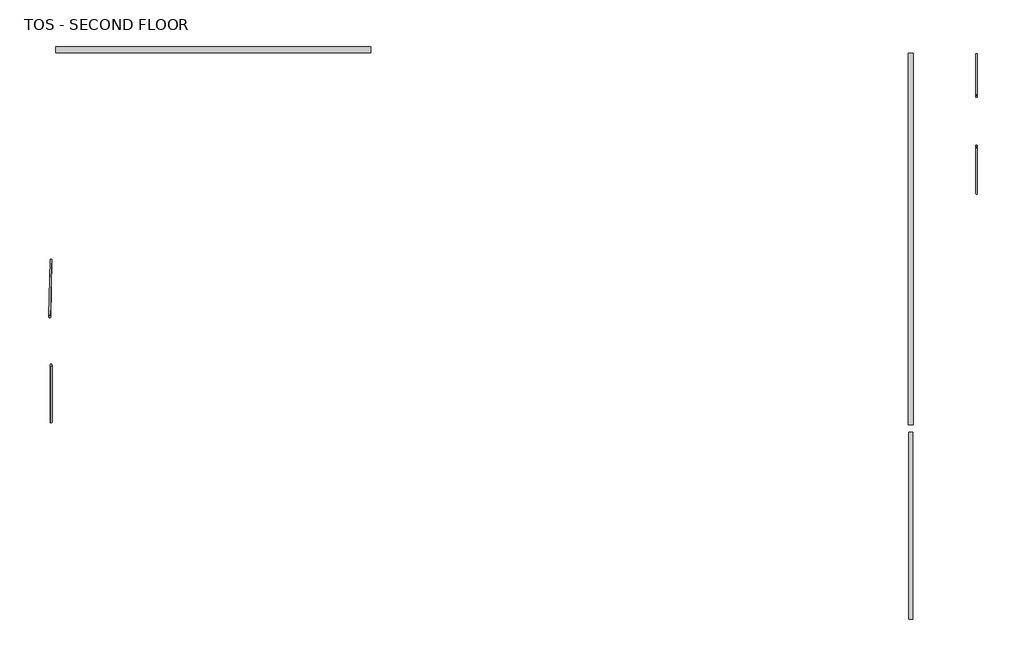
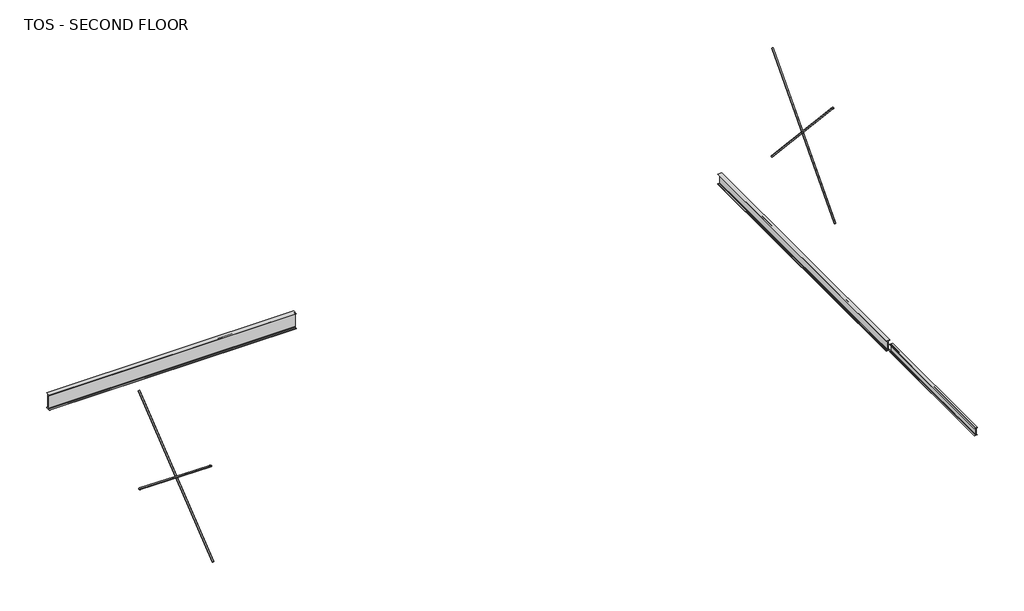
# One storey: 4 members, 3 beams.
"""IFC4 building model written with IfcOpenShell, lengths in millimetres."""

import ifcopenshell
import ifcopenshell.guid

model = None  # the IFC model being written
_history = None  # IfcOwnerHistory: only IFC2X3 demands one
_inside = {}  # id of a spatial element -> (the spatial element, [elements in it])
_under = {}  # id of a project, library or spatial element -> (it, [spatial elements below it])
_declared = {}  # id of a project -> (the project, [libraries it declares])
_typed = {}  # id of a type object -> (the type object, [elements of that type])
_made_of = {}  # id of a material, layer set ... -> (it, [elements and type objects made of it])


def new_model(schema):
    """Start an empty IFC model of exactly this schema.

    Asked for "IFC4X3", IfcOpenShell would pick the latest addendum, in which some entities
    have other attributes; the version numbers below select the first issue.
    IFC2X3 requires an IfcOwnerHistory on every rooted entity: one is made here for all.
    """
    global model, _history
    if schema == "IFC4X3":
        model = ifcopenshell.file(schema_version=(4, 3, 0, 0))
    else:
        model = ifcopenshell.file(schema=schema)
    _inside.clear()
    _under.clear()
    _declared.clear()
    _typed.clear()
    _made_of.clear()
    _history = None
    if model.schema == "IFC2X3":
        org = make("IfcOrganization", Name="unknown")
        user = make(
            "IfcPersonAndOrganization",
            ThePerson=make("IfcPerson", FamilyName="unknown"),
            TheOrganization=org,
        )
        app = make(
            "IfcApplication",
            ApplicationDeveloper=org,
            Version="unknown",
            ApplicationFullName="unknown",
            ApplicationIdentifier="unknown",
        )
        _history = make(
            "IfcOwnerHistory",
            OwningUser=user,
            OwningApplication=app,
            ChangeAction="ADDED",
            CreationDate=0,
        )
    return model


def make(cls, **values):
    """One entity of the class cls with the attributes given. An attribute that is None is left unset."""
    return model.create_entity(
        cls, **{name: value for name, value in values.items() if value is not None}
    )


def rooted(cls, **values):
    """An entity with a GlobalId (a new one), such as an element, a storey or a relation."""
    return make(cls, GlobalId=ifcopenshell.guid.new(), OwnerHistory=_history, **values)


def si_unit(unit_type, name, prefix=None):
    """IfcSIUnit, for example si_unit("LENGTHUNIT", "METRE", prefix="MILLI")."""
    return make("IfcSIUnit", UnitType=unit_type, Prefix=prefix, Name=name)


def assignment(units):
    """IfcUnitAssignment: the units of a project."""
    return None if units is None else make("IfcUnitAssignment", Units=units)


def point(xyz):
    """IfcCartesianPoint."""
    return None if xyz is None else make("IfcCartesianPoint", Coordinates=xyz)


def direction(xyz):
    """IfcDirection."""
    return None if xyz is None else make("IfcDirection", DirectionRatios=xyz)


def frame(location, z_axis=None, x_axis=None):
    """IfcAxis2Placement3D, a coordinate frame: its origin and axes. An axis left out is left unset."""
    return make(
        "IfcAxis2Placement3D",
        Location=point(location),
        Axis=direction(z_axis),
        RefDirection=direction(x_axis),
    )


def frame_2d(location, x_axis=None):
    """IfcAxis2Placement2D, a coordinate frame in the plane: its origin and x axis."""
    return make(
        "IfcAxis2Placement2D", Location=point(location), RefDirection=direction(x_axis)
    )


def origin():
    """The frame at (0, 0, 0) with its axes left unset."""
    return frame((0.0, 0.0, 0.0))


def origin_2d():
    """The frame at (0, 0) in the plane with its x axis left unset."""
    return frame_2d((0.0, 0.0))


def place(relative_to, where):
    """IfcLocalPlacement: puts the frame where relative to a parent placement (None: the world)."""
    return make(
        "IfcLocalPlacement", PlacementRelTo=relative_to, RelativePlacement=where
    )


def context(
    kind, dimensions, precision=None, world=None, true_north=None, identifier=None
):
    """IfcGeometricRepresentationContext, for example the 3D "Model" context."""
    return make(
        "IfcGeometricRepresentationContext",
        ContextIdentifier=identifier,
        ContextType=kind,
        CoordinateSpaceDimension=dimensions,
        Precision=precision,
        WorldCoordinateSystem=world,
        TrueNorth=true_north,
    )


def project(units=None, contexts=None):
    """IfcProject with its units and contexts."""
    return rooted(
        "IfcProject",
        Name="project",
        RepresentationContexts=contexts,
        UnitsInContext=assignment(units),
    )


def spatial(cls, under=None, at=None, **own):
    """A site, building, storey or space (cls), placed at a placement, below another one or the project."""
    s = rooted(cls, ObjectPlacement=at, **own)
    if under is not None:
        _under.setdefault(under.id(), (under, []))[1].append(s)
    return s


def polyline(points):
    """IfcPolyline through the points."""
    return make("IfcPolyline", Points=[point(p) for p in points])


def circle_curve(where, radius):
    """IfcCircle in the frame where."""
    return make("IfcCircle", Position=where, Radius=radius)


def trimmed(basis, trim1, trim2, sense, master):
    """IfcTrimmedCurve: the piece of a basis curve between two trims."""
    return make(
        "IfcTrimmedCurve",
        BasisCurve=basis,
        Trim1=trim1,
        Trim2=trim2,
        SenseAgreement=sense,
        MasterRepresentation=master,
    )


def segment(curve, same_sense, transition):
    """IfcCompositeCurveSegment."""
    return make(
        "IfcCompositeCurveSegment",
        Transition=transition,
        SameSense=same_sense,
        ParentCurve=curve,
    )


def composite_curve(segments, self_intersect=None):
    """IfcCompositeCurve: segments joined end to end."""
    return make("IfcCompositeCurve", Segments=segments, SelfIntersect=self_intersect)


def outline(outer, holes=None, kind="AREA"):
    """IfcArbitraryClosedProfileDef: a profile drawn as a closed curve; with holes, ...WithVoids."""
    if holes is None:
        return make("IfcArbitraryClosedProfileDef", ProfileType=kind, OuterCurve=outer)
    return make(
        "IfcArbitraryProfileDefWithVoids",
        ProfileType=kind,
        OuterCurve=outer,
        InnerCurves=holes,
    )


def extrude(swept, where, along, depth):
    """IfcExtrudedAreaSolid: the profile swept, set in the frame where, extruded along a direction by depth."""
    return make(
        "IfcExtrudedAreaSolid",
        SweptArea=swept,
        Position=where,
        ExtrudedDirection=direction(along),
        Depth=depth,
    )


def shape(context_of_items, identifier, shape_type, items):
    """IfcShapeRepresentation: the items that make up one representation, for example the "Body"."""
    return make(
        "IfcShapeRepresentation",
        ContextOfItems=context_of_items,
        RepresentationIdentifier=identifier,
        RepresentationType=shape_type,
        Items=items,
    )


def source(mapping_origin, context_of_items, identifier, shape_type, items):
    """IfcRepresentationMap: a shape defined once, which mapped items show again and again."""
    return make(
        "IfcRepresentationMap",
        MappingOrigin=mapping_origin,
        MappedRepresentation=shape(context_of_items, identifier, shape_type, items),
    )


def transform(
    local_origin,
    x_axis=None,
    y_axis=None,
    z_axis=None,
    scale=None,
    scale2=None,
    scale3=None,
    uniform=True,
):
    """IfcCartesianTransformationOperator3D, or its non-uniform kind. x_axis, y_axis, z_axis: its Axis1, 2, 3."""
    if uniform:
        return make(
            "IfcCartesianTransformationOperator3D",
            Axis1=direction(x_axis),
            Axis2=direction(y_axis),
            LocalOrigin=point(local_origin),
            Scale=scale,
            Axis3=direction(z_axis),
        )
    return make(
        "IfcCartesianTransformationOperator3DnonUniform",
        Axis1=direction(x_axis),
        Axis2=direction(y_axis),
        LocalOrigin=point(local_origin),
        Scale=scale,
        Axis3=direction(z_axis),
        Scale2=scale2,
        Scale3=scale3,
    )


def mapped(mapping_source, mapping_target):
    """IfcMappedItem: shows the shape of a source again, moved by a transform."""
    return make(
        "IfcMappedItem", MappingSource=mapping_source, MappingTarget=mapping_target
    )


def made_of(thing, what):
    """Note that an element or type object is made of a material, layer set ...; save() writes the relation."""
    if what is not None:
        _made_of.setdefault(what.id(), (what, []))[1].append(thing)
    return thing


def element(
    cls,
    number,
    at=None,
    inside=None,
    cuts=None,
    type_object=None,
    material=None,
    context=None,
    identifier="Body",
    shape_type=None,
    held_by="IfcProductDefinitionShape",
    body=None,
    shapes=None,
    **own,
):
    """One element of the class cls, such as IfcWall. Its Tag is "e" and its number.

    at: its placement. inside: the storey or other place that contains it. cuts: it is an
    opening in that element (IfcRelVoidsElement). A single representation is given by context,
    identifier, shape_type and body (its items); several are given by shapes. held_by: the class
    of the entity that holds the representations. save() writes the other relations.
    """
    e = rooted(cls, Tag="e%d" % number, ObjectPlacement=at, **own)
    if body is not None:
        shapes = [shape(context, identifier, shape_type, body)]
    if shapes is not None:
        e.Representation = make(held_by, Representations=shapes)
    if inside is not None:
        _inside.setdefault(inside.id(), (inside, []))[1].append(e)
    if cuts is not None:
        rooted(
            "IfcRelVoidsElement", RelatingBuildingElement=cuts, RelatedOpeningElement=e
        )
    if type_object is not None:
        _typed.setdefault(type_object.id(), (type_object, []))[1].append(e)
    return made_of(e, material)


def aggregate(whole, parts):
    """IfcRelAggregates: a whole, such as a stair, and the parts it consists of."""
    return rooted("IfcRelAggregates", RelatingObject=whole, RelatedObjects=parts)


def save(model, path):
    """Write the relations noted so far, then the file.

    IfcRelAggregates (storeys below a building ...), IfcRelContainedInSpatialStructure (elements
    in a storey), IfcRelDefinesByType, IfcRelAssociatesMaterial and IfcRelDeclares: one each for
    every whole, place, type object, material and project.
    """
    for whole, parts in _under.values():
        aggregate(whole, parts)
    for where, things in _inside.values():
        rooted(
            "IfcRelContainedInSpatialStructure",
            RelatedElements=things,
            RelatingStructure=where,
        )
    for kind, things in _typed.values():
        rooted("IfcRelDefinesByType", RelatedObjects=things, RelatingType=kind)
    for what, things in _made_of.values():
        rooted("IfcRelAssociatesMaterial", RelatedObjects=things, RelatingMaterial=what)
    for by, libraries in _declared.values():
        rooted("IfcRelDeclares", RelatingContext=by, RelatedDefinitions=libraries)
    model.write(path)


def w_wide_flange_w10x12_1bd4f99f(model_context):
    return source(origin(), model_context, "Body", "SweptSolid", [
        extrude(outline(composite_curve([segment(polyline([(50.292, -120.015), (50.292, -125.349), (-50.292, -125.349), (-50.292, -120.015), (-16.129, -120.015)]), True, "CONTINUOUS"), segment(trimmed(circle_curve(frame_2d((-16.129, -106.299)), 13.716), [point((-16.129, -120.015))], [point((-2.413, -106.299))], True, "CARTESIAN"), True, "CONTINUOUS"), segment(polyline([(-2.413, -106.299), (-2.413, 106.299)]), True, "CONTINUOUS"), segment(trimmed(circle_curve(frame_2d((-16.129, 106.299)), 13.716), [point((-2.413, 106.299))], [point((-16.129, 120.015))], True, "CARTESIAN"), True, "CONTINUOUS"), segment(polyline([(-16.129, 120.015), (-50.292, 120.015), (-50.292, 125.349), (50.292, 125.349), (50.292, 120.015), (16.129, 120.015)]), True, "CONTINUOUS"), segment(trimmed(circle_curve(frame_2d((16.129, 106.299)), 13.716), [point((16.129, 120.015))], [point((2.413, 106.299))], True, "CARTESIAN"), True, "CONTINUOUS"), segment(polyline([(2.413, 106.299), (2.413, -106.299)]), True, "CONTINUOUS"), segment(trimmed(circle_curve(frame_2d((16.129, -106.299)), 13.716), [point((2.413, -106.299))], [point((16.129, -120.015))], True, "CARTESIAN"), True, "CONTINUOUS"), segment(polyline([(16.129, -120.015), (50.292, -120.015)]), True, "CONTINUOUS")], self_intersect=False)), frame((-2408.2375, 0.0, 0.0), z_axis=(1.0, 0.0, 0.0), x_axis=(0.0, 1.0, 0.0)), (0.0, 0.0, 1.0), 4828.794),
    ])


def w_wide_flange_w14x22_9bef81b0(model_context):
    return source(origin(), model_context, "Body", "SweptSolid", [
        extrude(outline(composite_curve([segment(polyline([(63.5, -165.481), (63.5, -173.99), (-63.5, -173.99), (-63.5, -165.481), (-21.3995, -165.481)]), True, "CONTINUOUS"), segment(trimmed(circle_curve(frame_2d((-21.3995, -147.0025)), 18.4785), [point((-21.3995, -165.481))], [point((-2.921, -147.0025))], True, "CARTESIAN"), True, "CONTINUOUS"), segment(polyline([(-2.921, -147.0025), (-2.921, 147.0025)]), True, "CONTINUOUS"), segment(trimmed(circle_curve(frame_2d((-21.3995, 147.0025)), 18.4785), [point((-2.921, 147.0025))], [point((-21.3995, 165.481))], True, "CARTESIAN"), True, "CONTINUOUS"), segment(polyline([(-21.3995, 165.481), (-63.5, 165.481), (-63.5, 173.99), (63.5, 173.99), (63.5, 165.481), (21.3995, 165.481)]), True, "CONTINUOUS"), segment(trimmed(circle_curve(frame_2d((21.3995, 147.0025)), 18.4785), [point((21.3995, 165.481))], [point((2.921, 147.0025))], True, "CARTESIAN"), True, "CONTINUOUS"), segment(polyline([(2.921, 147.0025), (2.921, -147.0025)]), True, "CONTINUOUS"), segment(trimmed(circle_curve(frame_2d((21.3995, -147.0025)), 18.4785), [point((2.921, -147.0025))], [point((21.3995, -165.481))], True, "CARTESIAN"), True, "CONTINUOUS"), segment(polyline([(21.3995, -165.481), (63.5, -165.481)]), True, "CONTINUOUS")], self_intersect=False)), frame((-4799.838, 0.0, 0.0), z_axis=(1.0, 0.0, 0.0), x_axis=(0.0, 1.0, 0.0)), (0.0, 0.0, 1.0), 9594.088),
    ])


def w_wide_flange_w21x44_ac43757c(model_context):
    return source(origin(), model_context, "Body", "SweptSolid", [
        extrude(outline(composite_curve([segment(polyline([(82.55, -251.46), (82.55, -262.89), (-82.55, -262.89), (-82.55, -251.46), (-21.59, -251.46)]), True, "CONTINUOUS"), segment(trimmed(circle_curve(frame_2d((-21.59, -234.315)), 17.145), [point((-21.59, -251.46))], [point((-4.445, -234.315))], True, "CARTESIAN"), True, "CONTINUOUS"), segment(polyline([(-4.445, -234.315), (-4.445, 234.315)]), True, "CONTINUOUS"), segment(trimmed(circle_curve(frame_2d((-21.59, 234.315)), 17.145), [point((-4.445, 234.315))], [point((-21.59, 251.46))], True, "CARTESIAN"), True, "CONTINUOUS"), segment(polyline([(-21.59, 251.46), (-82.55, 251.46), (-82.55, 262.89), (82.55, 262.89), (82.55, 251.46), (21.59, 251.46)]), True, "CONTINUOUS"), segment(trimmed(circle_curve(frame_2d((21.59, 234.315)), 17.145), [point((21.59, 251.46))], [point((4.445, 234.315))], True, "CARTESIAN"), True, "CONTINUOUS"), segment(polyline([(4.445, 234.315), (4.445, -234.315)]), True, "CONTINUOUS"), segment(trimmed(circle_curve(frame_2d((21.59, -234.315)), 17.145), [point((4.445, -234.315))], [point((21.59, -251.46))], True, "CARTESIAN"), True, "CONTINUOUS"), segment(polyline([(21.59, -251.46), (82.55, -251.46)]), True, "CONTINUOUS")], self_intersect=False)), frame((-4105.2253906, 0.0, 0.0), z_axis=(1.0, 0.0, 0.0), x_axis=(0.0, 1.0, 0.0)), (0.0, 0.0, 1.0), 8138.2195313),
    ])


def hss_round_structural_tubing_hss1_900x0_188_a00ff317(model_context):
    return source(origin(), model_context, "Body", "SweptSolid", [
        extrude(outline(composite_curve([segment(trimmed(circle_curve(origin_2d(), 24.13), [point((-24.13, 0.0))], [point((24.13, 0.0))], False, "CARTESIAN"), True, "CONTINUOUS"), segment(trimmed(circle_curve(origin_2d(), 24.13), [point((24.13, 0.0))], [point((-24.13, 0.0))], False, "CARTESIAN"), True, "CONTINUOUS")], self_intersect=False), holes=[composite_curve([segment(trimmed(circle_curve(origin_2d(), 19.7104), [point((19.7104, 0.0))], [point((-19.7104, 0.0))], True, "CARTESIAN"), True, "CONTINUOUS"), segment(trimmed(circle_curve(origin_2d(), 19.7104), [point((-19.7104, 0.0))], [point((19.7104, 0.0))], True, "CARTESIAN"), True, "CONTINUOUS")], self_intersect=False)]), frame((-2686.9909588, 0.0, 0.0), z_axis=(1.0, 0.0, 0.0), x_axis=(0.0, 1.0, 0.0)), (0.0, 0.0, 1.0), 5419.7697281),
    ])


def hss_round_structural_tubing_hss1_900x0_188_38155dc2(model_context):
    return source(origin(), model_context, "Body", "SweptSolid", [
        extrude(outline(composite_curve([segment(trimmed(circle_curve(origin_2d(), 24.13), [point((-24.13, 0.0))], [point((24.13, 0.0))], False, "CARTESIAN"), True, "CONTINUOUS"), segment(trimmed(circle_curve(origin_2d(), 24.13), [point((24.13, 0.0))], [point((-24.13, 0.0))], False, "CARTESIAN"), True, "CONTINUOUS")], self_intersect=False), holes=[composite_curve([segment(trimmed(circle_curve(origin_2d(), 19.7104), [point((19.7104, 0.0))], [point((-19.7104, 0.0))], True, "CARTESIAN"), True, "CONTINUOUS"), segment(trimmed(circle_curve(origin_2d(), 19.7104), [point((-19.7104, 0.0))], [point((19.7104, 0.0))], True, "CARTESIAN"), True, "CONTINUOUS")], self_intersect=False)]), frame((-2686.9909377, 0.0, 0.0), z_axis=(1.0, 0.0, 0.0), x_axis=(0.0, 1.0, 0.0)), (0.0, 0.0, 1.0), 5419.0802818),
    ])


def hss_round_structural_tubing_hss1_900x0_188_139ededb(model_context):
    return source(origin(), model_context, "Body", "SweptSolid", [
        extrude(outline(composite_curve([segment(trimmed(circle_curve(origin_2d(), 24.13), [point((-24.13, 0.0))], [point((24.13, 0.0))], False, "CARTESIAN"), True, "CONTINUOUS"), segment(trimmed(circle_curve(origin_2d(), 24.13), [point((24.13, 0.0))], [point((-24.13, 0.0))], False, "CARTESIAN"), True, "CONTINUOUS")], self_intersect=False), holes=[composite_curve([segment(trimmed(circle_curve(origin_2d(), 19.7104), [point((19.7104, 0.0))], [point((-19.7104, 0.0))], True, "CARTESIAN"), True, "CONTINUOUS"), segment(trimmed(circle_curve(origin_2d(), 19.7104), [point((-19.7104, 0.0))], [point((19.7104, 0.0))], True, "CARTESIAN"), True, "CONTINUOUS")], self_intersect=False)]), frame((-2747.8254285, 0.0, 0.0), z_axis=(1.0, 0.0, 0.0), x_axis=(0.0, 1.0, 0.0)), (0.0, 0.0, 1.0), 5329.4064562),
    ])


def hss_round_structural_tubing_hss1_900x0_188_b26e8f7a(model_context):
    return source(origin(), model_context, "Body", "SweptSolid", [
        extrude(outline(composite_curve([segment(trimmed(circle_curve(origin_2d(), 24.13), [point((-24.13, 0.0))], [point((24.13, 0.0))], False, "CARTESIAN"), True, "CONTINUOUS"), segment(trimmed(circle_curve(origin_2d(), 24.13), [point((24.13, 0.0))], [point((-24.13, 0.0))], False, "CARTESIAN"), True, "CONTINUOUS")], self_intersect=False), holes=[composite_curve([segment(trimmed(circle_curve(origin_2d(), 19.7104), [point((19.7104, 0.0))], [point((-19.7104, 0.0))], True, "CARTESIAN"), True, "CONTINUOUS"), segment(trimmed(circle_curve(origin_2d(), 19.7104), [point((-19.7104, 0.0))], [point((19.7104, 0.0))], True, "CARTESIAN"), True, "CONTINUOUS")], self_intersect=False)]), frame((-2585.8479774, 0.0, 0.0), z_axis=(1.0, 0.0, 0.0), x_axis=(0.0, 1.0, 0.0)), (0.0, 0.0, 1.0), 5139.611762),
    ])


model = new_model("IFC4")

# Units and contexts
model_context = context("Model", 3, world=origin())
ifc_project = project(units=[si_unit("LENGTHUNIT", "METRE", prefix="MILLI")], contexts=[model_context])

# Site, building, storey
site = spatial("IfcSite", under=ifc_project)
building = spatial("IfcBuilding", under=site)
storey = spatial("IfcBuildingStorey", under=building, Name="TOS - SECOND FLOOR", Elevation=34378.9)

# Beams
placement = place(None, origin())
w_wide_flange_w10x12_shape = w_wide_flange_w10x12_1bd4f99f(model_context)
element("IfcBeam", 1, ObjectType="W-Wide Flange : W10X12", at=placement, inside=storey, context=model_context, shape_type="MappedRepresentation", body=[
    mapped(w_wide_flange_w10x12_shape, transform((11866.458706, -4439.2429995, 34253.551), x_axis=(0.0, -1.0, 0.0), y_axis=(1.0, 0.0, 0.0), z_axis=(0.0, 0.0, 1.0))),
])
w_wide_flange_w14x22_shape = w_wide_flange_w14x22_9bef81b0(model_context)
element("IfcBeam", 2, ObjectType="W-Wide Flange : W14X22", at=placement, inside=storey, context=model_context, shape_type="MappedRepresentation", body=[
    mapped(w_wide_flange_w14x22_shape, transform((11866.458706, 2953.7445005, 34204.91), x_axis=(0.0, -1.0, 0.0), y_axis=(1.0, 0.0, 0.0), z_axis=(0.0, 0.0, 1.0))),
])
w_wide_flange_w21x44_shape = w_wide_flange_w21x44_ac43757c(model_context)
element("IfcBeam", 3, ObjectType="W-Wide Flange : W21X44", at=placement, inside=storey, context=model_context, shape_type="MappedRepresentation", body=[
    mapped(w_wide_flange_w21x44_shape, transform((-6107.7454607, 7843.2445005, 34116.01), x_axis=(1.0, 0.0, 0.0), y_axis=(0.0, 1.0, 0.0), z_axis=(0.0, 0.0, 1.0))),
])

# Members
hss_round_structural_tubing_hss1_900x0_188_shape = hss_round_structural_tubing_hss1_900x0_188_a00ff317(model_context)
element("IfcMember", 4, ObjectType="HSS-Round Structural Tubing : HSS1.900X0.188", at=placement, inside=storey, context=model_context, shape_type="MappedRepresentation", body=[
    mapped(hss_round_structural_tubing_hss1_900x0_188_shape, transform((-10327.3204607, 323.2570005, 36086.161), x_axis=(0.0, 0.7802907102049828, 0.6254169869517489), y_axis=(-1.0000000000000002, 0.0, 0.0), z_axis=(0.0, -0.6254169869517489, 0.7802907102049828))),
])
hss_round_structural_tubing_hss1_900x0_188_2_shape = hss_round_structural_tubing_hss1_900x0_188_38155dc2(model_context)
element("IfcMember", 5, ObjectType="HSS-Round Structural Tubing : HSS1.900X0.188", at=placement, inside=storey, context=model_context, shape_type="MappedRepresentation", body=[
    mapped(hss_round_structural_tubing_hss1_900x0_188_2_shape, transform((-10375.5045038, 323.7709636, 36086.161), x_axis=(-0.016643361427993504, -0.7801131871647976, 0.6254169918797853), y_axis=(0.9997724962134591, -0.021329693272745007, 0.0), z_axis=(0.013339952604359658, 0.6252747071459654, 0.7802907062550735))),
])
hss_round_structural_tubing_hss1_900x0_188_3_shape = hss_round_structural_tubing_hss1_900x0_188_139ededb(model_context)
element("IfcMember", 6, ObjectType="HSS-Round Structural Tubing : HSS1.900X0.188", at=placement, inside=storey, context=model_context, shape_type="MappedRepresentation", body=[
    mapped(hss_round_structural_tubing_hss1_900x0_188_3_shape, transform((13567.7295393, 5974.7570005, 36273.105), x_axis=(0.0, 0.6703732705277827, 0.7420240414985786), y_axis=(-1.0000000000000002, 0.0, 0.0), z_axis=(0.0, -0.7420240414985786, 0.6703732705277827))),
])
hss_round_structural_tubing_hss1_900x0_188_4_shape = hss_round_structural_tubing_hss1_900x0_188_b26e8f7a(model_context)
element("IfcMember", 7, ObjectType="HSS-Round Structural Tubing : HSS1.900X0.188", at=placement, inside=storey, context=model_context, shape_type="MappedRepresentation", body=[
    mapped(hss_round_structural_tubing_hss1_900x0_188_4_shape, transform((13567.7295393, 5974.7570005, 36308.411), x_axis=(0.0, -0.6767091971854916, 0.736250407432531), y_axis=(1.0000000000000002, 0.0, 0.0), z_axis=(0.0, 0.736250407432531, 0.6767091971854916))),
])

save(model, "model.ifc")

# Revit data of these elements
# Type "W-Wide Flange : W10X12"
#   Assembly Code = "B10"
#   W = 12
#   Length [instance default] = 1524 mm
#   bf = 100.584 mm
#   d = 250.698 mm
#   k = 19.05 mm
#   k2 = 13.716 mm
#   tf = 5.334 mm
#   tw = 4.826 mm
#   A = 0.00228387 m²
#   Structural Material [instance default] = Steel ASTM A992
# Type "W-Wide Flange : W14X22"
#   Assembly Code = "B10"
#   W = 22
#   Length [instance default] = 1524 mm
#   bf = 127 mm
#   d = 347.98 mm
#   k = 26.988 mm
#   k2 = 18.479 mm
#   tf = 8.509 mm
#   tw = 5.842 mm
#   A = 0.00418709 m²
#   Structural Material [instance default] = Steel ASTM A992
# Type "W-Wide Flange : W21X44"
#   Assembly Code = "B10"
#   W = 44
#   Length [instance default] = 1524 mm
#   bf = 165.1 mm
#   d = 525.78 mm
#   k = 28.575 mm
#   k2 = 17.145 mm
#   tf = 11.43 mm
#   tw = 8.89 mm
#   A = 0.00838708 m²
#   Structural Material [instance default] = Steel ASTM A992
# Type "HSS-Round Structural Tubing : HSS1.900X0.188"
#   Assembly Code = "B10"
#   t = 4.42 mm
#   W = 3.44
#   Length [instance default] = 1524 mm
#   OD = 48.26 mm
#   A = 0.000608386 m²
#   Structural Material [instance default] = Steel ASTM A500, Grade B, Round
# Element 1 (IfcBeam, "W-Wide Flange : W10X12")
#   Comments = ""
#   RM User Number = 62
#   RM Unique Id = 849
#   RS Unique Id = 274617
#   Structural Material = Aluminum, Anodized Red
#   Phase Created = New Construction
#   Materials on its faces: "Aluminum, Anodized Red"
# Element 2 (IfcBeam, "W-Wide Flange : W14X22")
#   Comments = ""
#   RM User Number = 58
#   RM Unique Id = 845
#   RS Unique Id = 274511
#   Structural Material = Aluminum, Anodized Red
#   Phase Created = New Construction
#   Materials on its faces: "Aluminum, Anodized Red"
# Element 3 (IfcBeam, "W-Wide Flange : W21X44")
#   Comments = ""
#   RM User Number = 17
#   RM Unique Id = 805
#   RS Unique Id = 272737
#   Structural Material = Aluminum, Anodized Red
#   Phase Created = New Construction
#   Materials on its faces: "Aluminum, Anodized Red"
# Element 4 (IfcMember, "HSS-Round Structural Tubing : HSS1.900X0.188")
#   Comments = ""
#   RM User Number = 94
#   RM Unique Id = 881
#   RS Unique Id = 276854
#   Phase Created = New Construction
#   Materials on its faces: "Steel ASTM A500, Grade B, Round"
# Element 5 (IfcMember, "HSS-Round Structural Tubing : HSS1.900X0.188")
#   Comments = ""
#   RM User Number = 93
#   RM Unique Id = 880
#   RS Unique Id = 276819
#   Phase Created = New Construction
#   Materials on its faces: "Steel ASTM A500, Grade B, Round"
# Element 6 (IfcMember, "HSS-Round Structural Tubing : HSS1.900X0.188")
#   Comments = ""
#   RM User Number = 115
#   RM Unique Id = 902
#   RS Unique Id = 287467
#   Phase Created = New Construction
#   Materials on its faces: "Steel ASTM A500, Grade B, Round"
# Element 7 (IfcMember, "HSS-Round Structural Tubing : HSS1.900X0.188")
#   Comments = ""
#   RM User Number = 116
#   RM Unique Id = 903
#   RS Unique Id = 287608
#   Phase Created = New Construction
#   Materials on its faces: "Steel ASTM A500, Grade B, Round"
# Materials
#   "Steel ASTM A992": class "Metal", colour RGB 128 0 0, transparency 0, Description = "Structural steel 50ksi", Cost = 0
#   "Steel ASTM A500, Grade B, Round": class "Metal", colour RGB 199 199 199, transparency 0, Description = "Carbon steel", Cost = 0
#   "Aluminum, Anodized Red": class "Metal", colour RGB 120 120 120, transparency 0, Description = "Anodized aluminum, red", Cost = 0
